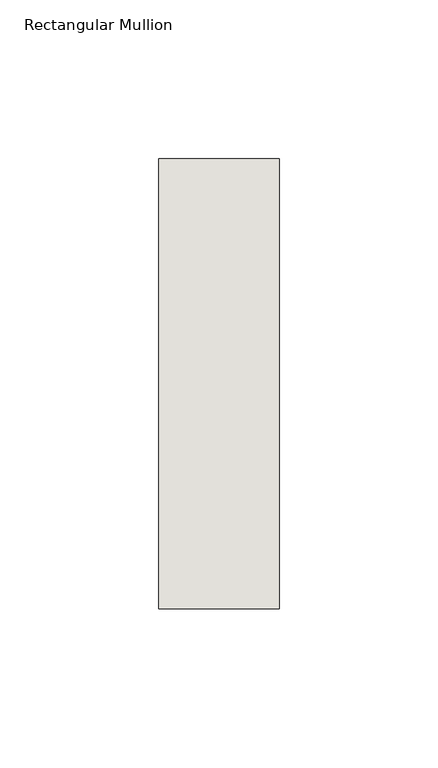
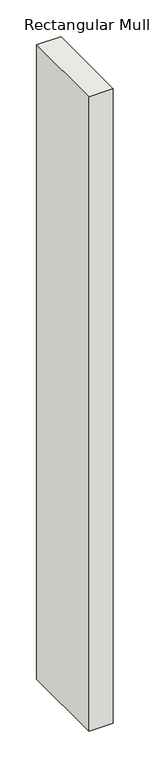
"""IFC4 building model written with IfcOpenShell, lengths in millimetres: wall geometry, Rectangular Mullion : NLRS_21_CWM_hsb-regel 38x142_gen_rsf."""

from ifc_helpers import new_model, si_unit, frame, origin, place, context, project, spatial, polyline, outline, extrude, source, transform, mapped, element, save


def rectangular_mullion_1165df42(model_context):
    return source(origin(), model_context, "Body", "SweptSolid", [
        extrude(outline(polyline([(-38.0, -71.0), (-38.0, 71.0), (0.0, 71.0), (0.0, -71.0), (-38.0, -71.0)])), frame((0.0, 0.0, -1050.0), z_axis=(0.0, 0.0, 1.0), x_axis=(1.0, 0.0, 0.0)), (0.0, 0.0, 1.0), 1050.0),
    ])


if __name__ == "__main__":
    model = new_model("IFC4")
    model_context = context("Model", 3, world=origin())
    ifc_project = project(units=[si_unit("LENGTHUNIT", "METRE", prefix="MILLI")], contexts=[model_context])
    site = spatial("IfcSite", under=ifc_project)
    building = spatial("IfcBuilding", under=site)
    placement = place(None, origin())
    rectangular_mullion_shape = rectangular_mullion_1165df42(model_context)
    element("IfcWall", 1, ObjectType="Rectangular Mullion : NLRS_21_CWM_hsb-regel 38x142_gen_rsf", at=placement, inside=building, context=model_context, shape_type="MappedRepresentation", body=[
        mapped(rectangular_mullion_shape, transform((0.0, 0.0, 0.0), x_axis=(1.0, 0.0, 0.0), y_axis=(0.0, 1.0, 0.0), z_axis=(0.0, 0.0, 1.0))),
    ])
    save(model, "model.ifc")

# Revit data of these elements
# Type "Rectangular Mullion : NLRS_21_CWM_hsb-regel 38x142_gen_rsf"
#   Type IfcGUID = "07M7mRoiH1CR8m_RSKIwpF"
#   Assembly Code = "21.10"
#   IfcExportAs = "IfcWall"
#   built-in parameter 1007322 = 0.465879 (stored number, unit not read)
#   built-in parameter 1007321 = 0.062336 (stored number, unit not read)
#   built-in parameter 1007320 = 0.062336 (stored number, unit not read)
# Element 1 (IfcWall, "Rectangular Mullion : NLRS_21_CWM_hsb-regel 38x142_gen_rsf")
#   Materials on its faces: "NLRS_i2_hout naaldhout vuren_gen_rsf"
# Materials
#   "NLRS_i2_hout naaldhout vuren_gen_rsf": class "I - Hout", colour RGB 234 199 147, transparency 0, Keynote = "i2", Manufacturer = "Revit Standards Foundation", URL = "www.revitstandards.org", Description = "hout vuren", Cost = 0
